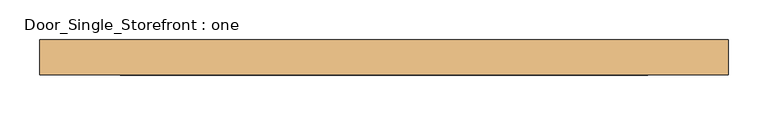
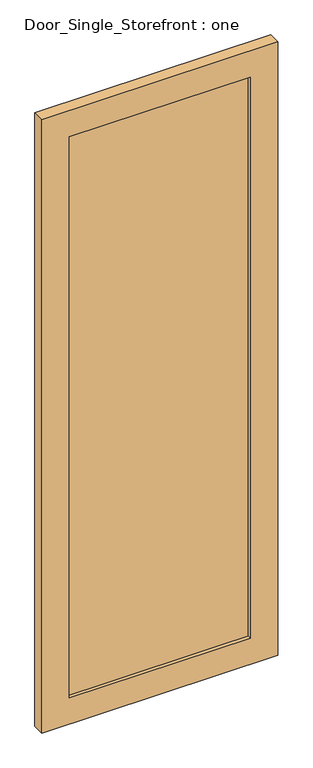
"""IFC4 building model written with IfcOpenShell, lengths in millimetres: door geometry, Door_Single_Storefront : one."""

from ifc_helpers import new_model, si_unit, frame, origin, place, context, project, spatial, polyline, outline, extrude, source, transform, mapped, element, save


def door_single_storefront_one_d6c5e293(model_context):
    return source(origin(), model_context, "Body", "SweptSolid", [
        extrude(outline(polyline([(2387.6, -434.18125), (0.0, -434.18125), (0.0, 434.18125), (2387.6, 434.18125), (2387.6, -434.18125)]), holes=[polyline([(101.6, 332.58125), (101.6, -332.58125), (2286.0, -332.58125), (2286.0, 332.58125), (101.6, 332.58125)])]), frame((0.0, 6.35, 0.0), z_axis=(0.0, 1.0, 0.0), x_axis=(0.0, 0.0, 1.0)), (0.0, 0.0, 1.0), 44.45),
        extrude(outline(polyline([(332.58125, 19.05), (-332.58125, 19.05), (-332.58125, 38.1), (332.58125, 38.1), (332.58125, 19.05)])), frame((0.0, 0.0, 101.6), z_axis=(0.0, 0.0, 1.0), x_axis=(1.0, 0.0, 0.0)), (0.0, 0.0, 1.0), 2184.4),
    ])


if __name__ == "__main__":
    model = new_model("IFC4")
    model_context = context("Model", 3, world=origin())
    ifc_project = project(units=[si_unit("LENGTHUNIT", "METRE", prefix="MILLI")], contexts=[model_context])
    site = spatial("IfcSite", under=ifc_project)
    building = spatial("IfcBuilding", under=site)
    placement = place(None, origin())
    door_single_storefront_one_shape = door_single_storefront_one_d6c5e293(model_context)
    element("IfcDoor", 1, ObjectType="Door_Single_Storefront : one", at=placement, inside=building, context=model_context, shape_type="MappedRepresentation", body=[
        mapped(door_single_storefront_one_shape, transform((0.0, 0.0, 0.0), x_axis=(1.0, 0.0, 0.0), y_axis=(0.0, 1.0, 0.0), z_axis=(0.0, 0.0, 1.0))),
    ])
    save(model, "model.ifc")

# Revit data of these elements
# Type "Door_Single_Storefront : one"
#   Type Mark = "27"
#   Analytic Construction = "<None>"
#   Stile_Width = 0' - 4"
#   Door_Thickness = 0' - 1 3/4"
#   Door_Offset = 0' - 2"
#   Glass_Material = Glass
#   Frame_Material = Aluminum
#   Function = (empty or 0)
# Element 1 (IfcDoor, "Door_Single_Storefront : one")
#   Materials on its faces: "Aluminum", "Glass"
# Materials
#   "Glass": class "Glass", colour RGB 0 128 192, transparency 0.75, Description = "Soda Lime Glass", Cost = 0
#   "Aluminum": class "Metal", colour RGB 247 247 247, transparency 0, Description = "Aluminum 6061", Cost = 0
